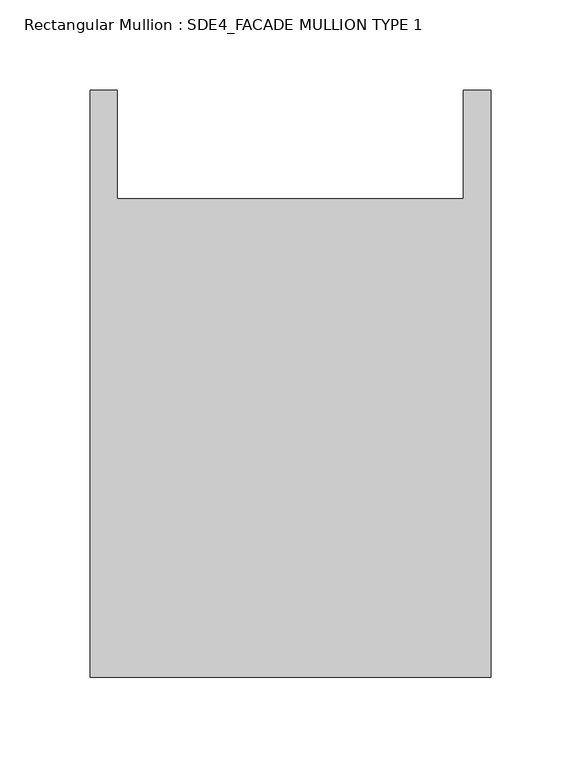
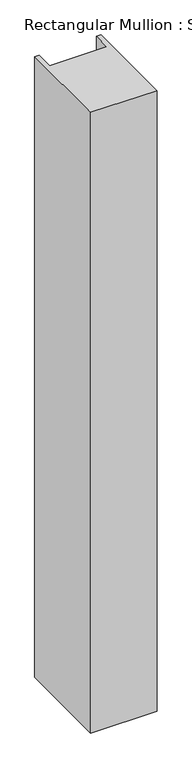
"""IFC4 building model written with IfcOpenShell, lengths in millimetres: member geometry, Rectangular Mullion : SDE4_FACADE MULLION TYPE 1."""

from ifc_helpers import new_model, si_unit, frame, origin, place, context, project, spatial, polyline, outline, extrude, source, transform, mapped, element, save


def rectangular_mullion_sde4_facade_mullion_type_1_72ac443e(model_context):
    return source(origin(), model_context, "Body", "SweptSolid", [
        extrude(outline(polyline([(111.0, -132.5), (-111.0, -132.5), (-111.0, 192.5), (-96.0, 192.5), (-96.0, 132.5), (96.0, 132.5), (96.0, 192.5), (111.0, 192.5), (111.0, -132.5)])), frame((0.0, 0.0, -2199.5956314), z_axis=(0.0, 0.0, 1.0), x_axis=(1.0, 0.0, 0.0)), (0.0, 0.0, 1.0), 2199.5956314),
    ])


if __name__ == "__main__":
    model = new_model("IFC4")
    model_context = context("Model", 3, world=origin())
    ifc_project = project(units=[si_unit("LENGTHUNIT", "METRE", prefix="MILLI")], contexts=[model_context])
    site = spatial("IfcSite", under=ifc_project)
    building = spatial("IfcBuilding", under=site)
    placement = place(None, origin())
    rectangular_mullion_sde4_facade_mullion_type_1_shape = rectangular_mullion_sde4_facade_mullion_type_1_72ac443e(model_context)
    element("IfcMember", 1, ObjectType="Rectangular Mullion : SDE4_FACADE MULLION TYPE 1", at=placement, inside=building, context=model_context, shape_type="MappedRepresentation", body=[
        mapped(rectangular_mullion_sde4_facade_mullion_type_1_shape, transform((0.0, 0.0, 0.0), x_axis=(1.0, 0.0, 0.0), y_axis=(0.0, 1.0, 0.0), z_axis=(0.0, 0.0, 1.0))),
    ])
    save(model, "model.ifc")

# Revit data of these elements
# Type "Rectangular Mullion : SDE4_FACADE MULLION TYPE 1"
#   built-in parameter 1007322 = 0.869423 (stored number, unit not read)
#   built-in parameter 1007321 = 0.364173 (stored number, unit not read)
#   built-in parameter 1007320 = 0.364173 (stored number, unit not read)
